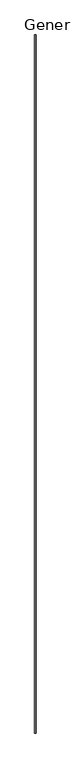
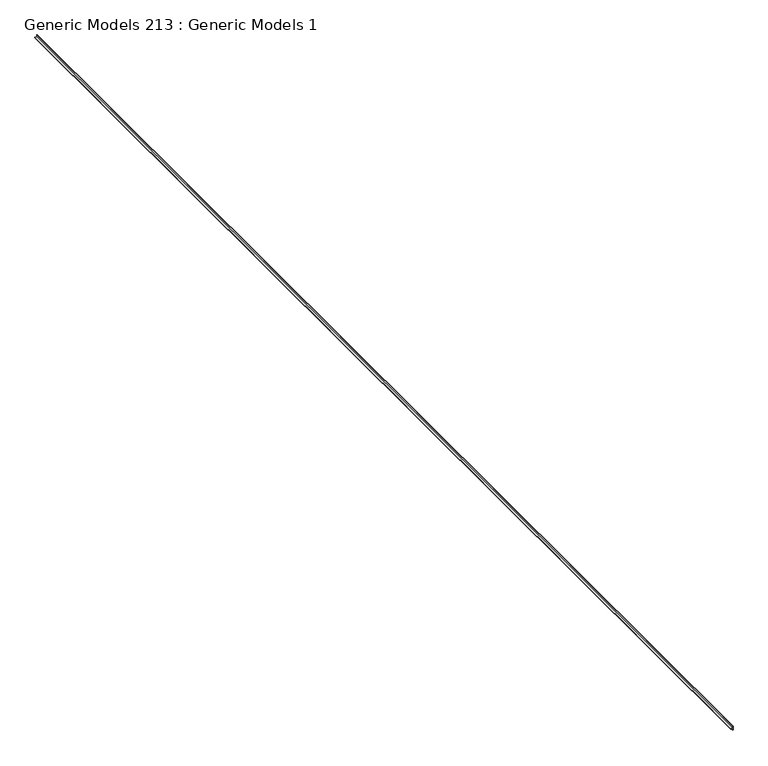
"""IFC4 building model written with IfcOpenShell, lengths in millimetres: proxy geometry, Generic Models 213 : Generic Models 1."""

from ifc_helpers import new_model, si_unit, frame, origin, place, context, project, spatial, polyline, outline, extrude, source, transform, mapped, element, save


def generic_models_213_generic_models_1_ced12685(model_context):
    return source(origin(), model_context, "Body", "SweptSolid", [
        extrude(outline(polyline([(126342.521, -6625.8562339), (126342.521, -6627.1262339), (126323.471, -6627.1262339), (126323.471, -6648.0812339), (126318.7212, -6648.0812339), (126318.7212, -6646.8112339), (126322.201, -6646.8112339), (126322.201, -6627.1262339), (126303.151, -6627.1262339), (126303.151, -6625.8562339), (126342.521, -6625.8562339)])), frame((0.0, -12706.9230338, 0.0), z_axis=(0.0, 1.0, 0.0), x_axis=(0.0, 0.0, 1.0)), (0.0, 0.0, 1.0), 12446.0),
    ])


if __name__ == "__main__":
    model = new_model("IFC4")
    model_context = context("Model", 3, world=origin())
    ifc_project = project(units=[si_unit("LENGTHUNIT", "METRE", prefix="MILLI")], contexts=[model_context])
    site = spatial("IfcSite", under=ifc_project)
    building = spatial("IfcBuilding", under=site)
    placement = place(None, origin())
    generic_models_213_generic_models_1_shape = generic_models_213_generic_models_1_ced12685(model_context)
    element("IfcBuildingElementProxy", 1, Name="Generic Models 213 : Generic Models 1", ObjectType="Generic Models 213 : Generic Models 1", at=placement, inside=building, context=model_context, shape_type="MappedRepresentation", body=[
        mapped(generic_models_213_generic_models_1_shape, transform((0.0, 0.0, 0.0), x_axis=(1.0, 0.0, 0.0), y_axis=(0.0, 1.0, 0.0), z_axis=(0.0, 0.0, 1.0))),
    ])
    save(model, "model.ifc")

# Revit data of these elements
# Element 1 (IfcBuildingElementProxy, "Generic Models 213 : Generic Models 1")
#   Materials on its faces: "_ 16 GA. COPPER VENTED T REVEAL BEAD (CONT. AROUND PERIMETER OF BEAM)"
# Materials
#   "_ 16 GA. COPPER VENTED T REVEAL BEAD (CONT. AROUND PERIMETER OF BEAM)": class "Generic", colour RGB 253 192 103, transparency 0, Cost = 0
